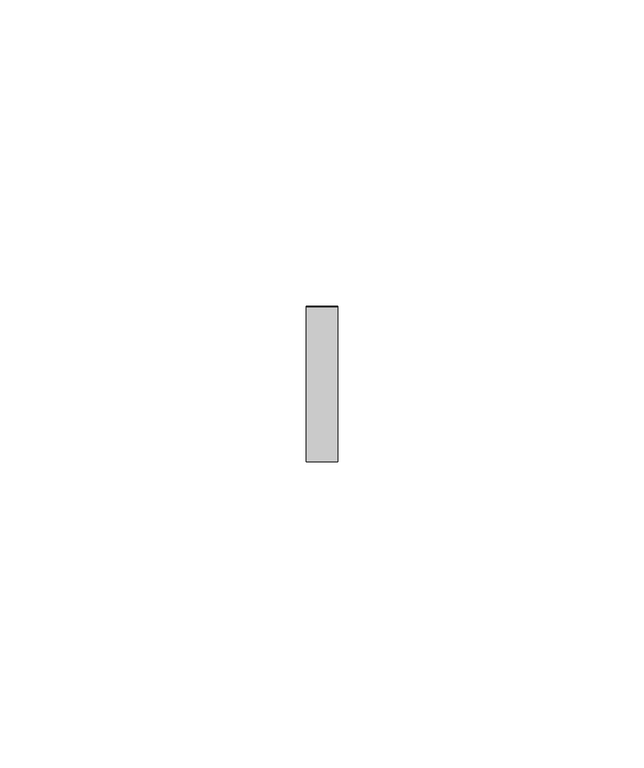
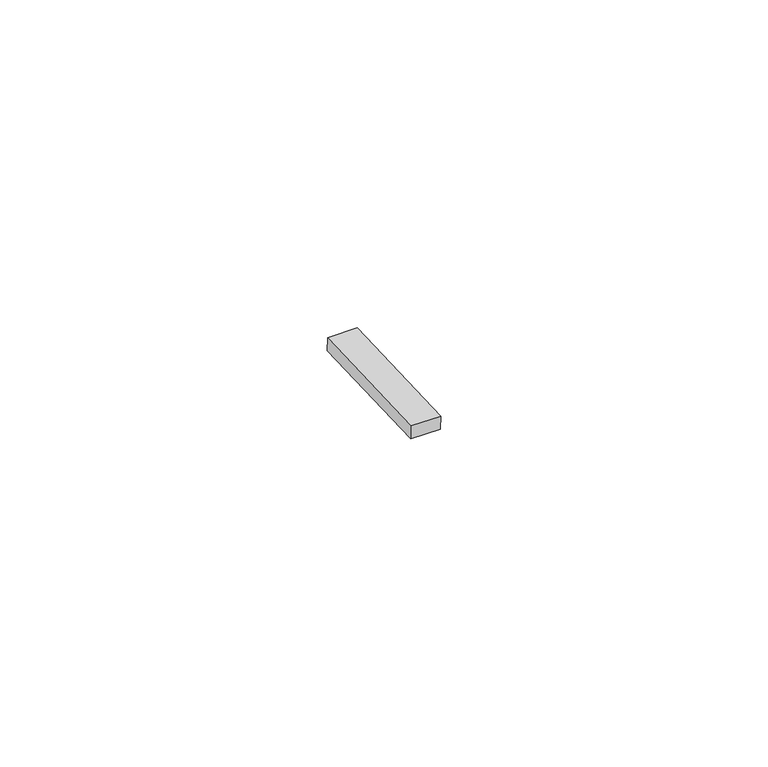
"""IFC4 building model written with IfcOpenShell, lengths in millimetres: proxy geometry, Inner panel:Inner panel:1:Inner panel:1 : Inner panel:Inner panel:300324:2:Inner panel:1:Inner panel:1 : Inner panel:Inner panel:300324:2 : Inner panel:Inner panel:1:Inner panel:1 : Inner panel:Inner panel:300324:300043:72 : Inner panel:Inner panel:1:Inner panel:1 : Inner panel:Inner panel:300324:2:Inner panel:1:Inner panel:1 : Inner panel:Inner panel:300324:2 : Inner panel:Inner panel:1:Inner panel:1 : Inner panel:Inner panel:300324:300043:308120."""

from ifc_helpers import new_model, si_unit, frame, origin, place, context, project, spatial, polyline, outline, extrude, source, transform, mapped, element, save


def generic_models_dd3bdfdf(model_context):
    return source(origin(), model_context, "Body", "SweptSolid", [
        extrude(outline(polyline([(0.0, -25.3999999), (0.0, 0.0), (5.2138089, 0.0), (5.2138089, -25.3999999), (0.0, -25.3999999)])), frame((592717.395117, -566905.6162814, 8857.0720004), z_axis=(0.0, -0.041630544712223896, 0.9991330730923502), x_axis=(-1.0, 0.0, 0.0)), (0.0, 0.0, 1.0), 2.4763745),
    ])


if __name__ == "__main__":
    model = new_model("IFC4")
    model_context = context("Model", 3, world=origin())
    ifc_project = project(units=[si_unit("LENGTHUNIT", "METRE", prefix="MILLI")], contexts=[model_context])
    site = spatial("IfcSite", under=ifc_project)
    building = spatial("IfcBuilding", under=site)
    placement = place(None, origin())
    generic_models_shape = generic_models_dd3bdfdf(model_context)
    element("IfcBuildingElementProxy", 1, Name="Inner panel:Inner panel:1:Inner panel:1 : Inner panel:Inner panel:300324:2:Inner panel:1:Inner panel:1 : Inner panel:Inner panel:300324:2 : Inner panel:Inner panel:1:Inner panel:1 : Inner panel:Inner panel:300324:300043:72 : Inner panel:Inner panel:1:Inner panel:1 : Inner panel:Inner panel:300324:2:Inner panel:1:Inner panel:1 : Inner panel:Inner panel:300324:2 : Inner panel:Inner panel:1:Inner panel:1 : Inner panel:Inner panel:300324:300043:308120", ObjectType="Inner panel:Inner panel:1:Inner panel:1 : Inner panel:Inner panel:300324:2:Inner panel:1:Inner panel:1 : Inner panel:Inner panel:300324:2 : Inner panel:Inner panel:1:Inner panel:1 : Inner panel:Inner panel:300324:300043:72 : Inner panel:Inner panel:1:Inner panel:1 : Inner panel:Inner panel:300324:2:Inner panel:1:Inner panel:1 : Inner panel:Inner panel:300324:2 : Inner panel:Inner panel:1:Inner panel:1 : Inner panel:Inner panel:300324:300043:308120", at=placement, inside=building, context=model_context, shape_type="MappedRepresentation", body=[
        mapped(generic_models_shape, transform((0.0, 0.0, 0.0), x_axis=(1.0, 0.0, 0.0), y_axis=(0.0, 1.0, 0.0), z_axis=(0.0, 0.0, 1.0))),
    ])
    save(model, "model.ifc")

# Revit data of these elements
# Type "Inner panel:Inner panel:1:Inner panel:1 : Inner panel:Inner panel:300324:2:Inner panel:1:Inner panel:1 : Inner panel:Inner panel:300324:2 : Inner panel:Inner panel:1:Inner panel:1 : Inner panel:Inner panel:300324:300043:72 : Inner panel:Inner panel:1:Inner panel:1 : Inner panel:Inner panel:300324:2:Inner panel:1:Inner panel:1 : Inner panel:Inner panel:300324:2 : Inner panel:Inner panel:1:Inner panel:1 : Inner panel:Inner panel:300324:300043:308120"
#   NameOverride = "Inner panel:Inner panel:1:Inner panel:1 : Inner panel:Inner panel:300324:2:Inner panel:1:Inner panel:1 : Inner panel:Inner panel:300324:2 : Inner panel:Inner panel:1:Inner panel:1 : Inner panel:Inner panel:300324:300043:308120"
#   ObjectTypeOverride = "Inner panel:1:Inner panel:1 : Inner panel:Inner panel:300324:2 : Inner panel:Inner panel:1:Inner panel:1 : Inner panel:Inner panel:300324:300043"
#   Reference = "Inner panel"
#   Tag = "308120"
# Element 1 (IfcBuildingElementProxy, "Inner panel:Inner panel:1:Inner panel:1 : Inner panel:Inner panel:300324:2:Inner panel:1:Inner panel:1 : Inner panel:Inner panel:300324:2 : Inner panel:Inner panel:1:Inner panel:1 : Inner panel:Inner panel:300324:300043:72 : Inner panel:Inner panel:1:Inner panel:1 : Inner panel:Inner panel:300324:2:Inner panel:1:Inner panel:1 : Inner panel:Inner panel:300324:2 : Inner panel:Inner panel:1:Inner panel:1 : Inner panel:Inner panel:300324:300043:308120")
#   Materials on its faces: "AT CLIP - 1\" WIDE NON ABSORBENT, WEATHER-RESISTANT NEOPRENE/EPDM/SBR FOAM"
# Materials
#   "AT CLIP - 1\" WIDE NON ABSORBENT, WEATHER-RESISTANT NEOPRENE/EPDM/SBR FOAM": class "Generic", colour RGB 85 85 85, transparency 0, Cost = 0
